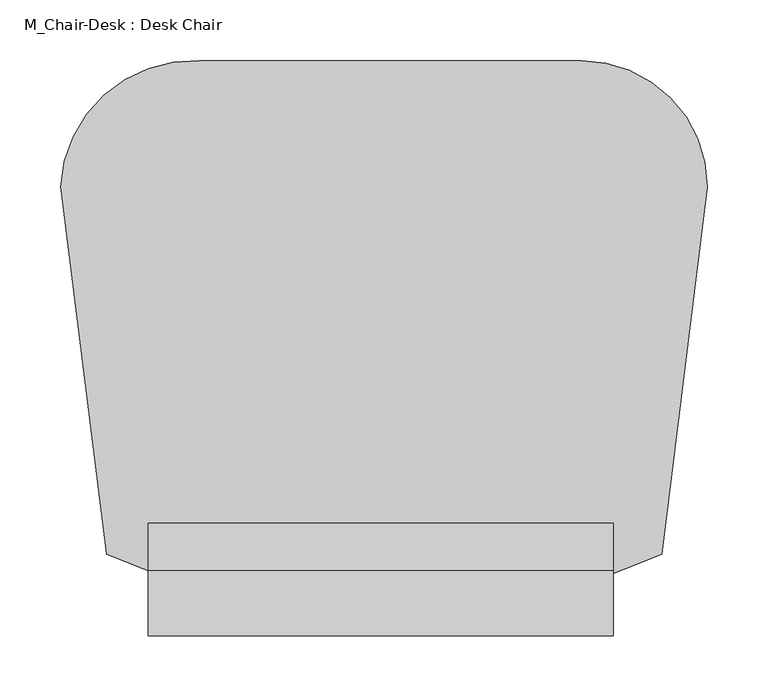
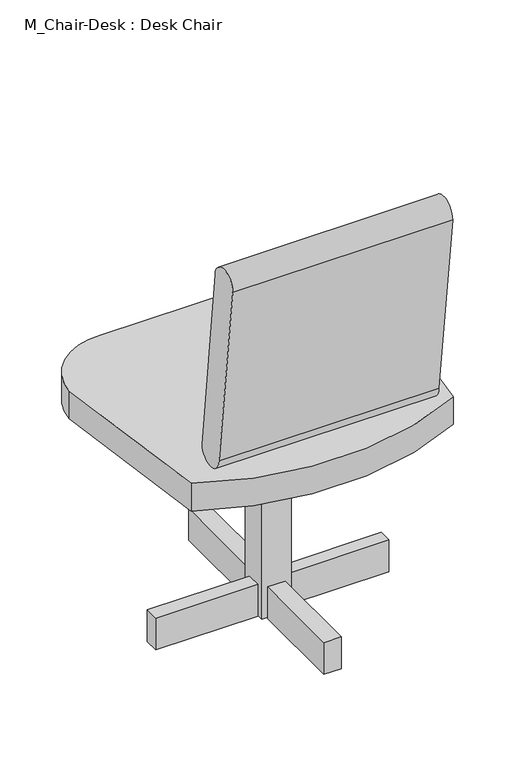
"""IFC4 building model written with IfcOpenShell, lengths in millimetres: furniture geometry, M_Chair-Desk : Desk Chair."""

import ifcopenshell
import ifcopenshell.guid

model = None  # the IFC model being written
_history = None  # IfcOwnerHistory: only IFC2X3 demands one
_inside = {}  # id of a spatial element -> (the spatial element, [elements in it])
_under = {}  # id of a project, library or spatial element -> (it, [spatial elements below it])
_declared = {}  # id of a project -> (the project, [libraries it declares])
_typed = {}  # id of a type object -> (the type object, [elements of that type])
_made_of = {}  # id of a material, layer set ... -> (it, [elements and type objects made of it])


def new_model(schema):
    """Start an empty IFC model of exactly this schema.

    Asked for "IFC4X3", IfcOpenShell would pick the latest addendum, in which some entities
    have other attributes; the version numbers below select the first issue.
    IFC2X3 requires an IfcOwnerHistory on every rooted entity: one is made here for all.
    """
    global model, _history
    if schema == "IFC4X3":
        model = ifcopenshell.file(schema_version=(4, 3, 0, 0))
    else:
        model = ifcopenshell.file(schema=schema)
    _inside.clear()
    _under.clear()
    _declared.clear()
    _typed.clear()
    _made_of.clear()
    _history = None
    if model.schema == "IFC2X3":
        org = make("IfcOrganization", Name="unknown")
        user = make(
            "IfcPersonAndOrganization",
            ThePerson=make("IfcPerson", FamilyName="unknown"),
            TheOrganization=org,
        )
        app = make(
            "IfcApplication",
            ApplicationDeveloper=org,
            Version="unknown",
            ApplicationFullName="unknown",
            ApplicationIdentifier="unknown",
        )
        _history = make(
            "IfcOwnerHistory",
            OwningUser=user,
            OwningApplication=app,
            ChangeAction="ADDED",
            CreationDate=0,
        )
    return model


def make(cls, **values):
    """One entity of the class cls with the attributes given. An attribute that is None is left unset."""
    return model.create_entity(
        cls, **{name: value for name, value in values.items() if value is not None}
    )


def rooted(cls, **values):
    """An entity with a GlobalId (a new one), such as an element, a storey or a relation."""
    return make(cls, GlobalId=ifcopenshell.guid.new(), OwnerHistory=_history, **values)


def si_unit(unit_type, name, prefix=None):
    """IfcSIUnit, for example si_unit("LENGTHUNIT", "METRE", prefix="MILLI")."""
    return make("IfcSIUnit", UnitType=unit_type, Prefix=prefix, Name=name)


def assignment(units):
    """IfcUnitAssignment: the units of a project."""
    return None if units is None else make("IfcUnitAssignment", Units=units)


def point(xyz):
    """IfcCartesianPoint."""
    return None if xyz is None else make("IfcCartesianPoint", Coordinates=xyz)


def direction(xyz):
    """IfcDirection."""
    return None if xyz is None else make("IfcDirection", DirectionRatios=xyz)


def frame(location, z_axis=None, x_axis=None):
    """IfcAxis2Placement3D, a coordinate frame: its origin and axes. An axis left out is left unset."""
    return make(
        "IfcAxis2Placement3D",
        Location=point(location),
        Axis=direction(z_axis),
        RefDirection=direction(x_axis),
    )


def frame_2d(location, x_axis=None):
    """IfcAxis2Placement2D, a coordinate frame in the plane: its origin and x axis."""
    return make(
        "IfcAxis2Placement2D", Location=point(location), RefDirection=direction(x_axis)
    )


def origin():
    """The frame at (0, 0, 0) with its axes left unset."""
    return frame((0.0, 0.0, 0.0))


def origin_with_axes():
    """The frame at (0, 0, 0) with the z axis (0, 0, 1) and the x axis (1, 0, 0) written out."""
    return frame((0.0, 0.0, 0.0), z_axis=(0.0, 0.0, 1.0), x_axis=(1.0, 0.0, 0.0))


def place(relative_to, where):
    """IfcLocalPlacement: puts the frame where relative to a parent placement (None: the world)."""
    return make(
        "IfcLocalPlacement", PlacementRelTo=relative_to, RelativePlacement=where
    )


def context(
    kind, dimensions, precision=None, world=None, true_north=None, identifier=None
):
    """IfcGeometricRepresentationContext, for example the 3D "Model" context."""
    return make(
        "IfcGeometricRepresentationContext",
        ContextIdentifier=identifier,
        ContextType=kind,
        CoordinateSpaceDimension=dimensions,
        Precision=precision,
        WorldCoordinateSystem=world,
        TrueNorth=true_north,
    )


def project(units=None, contexts=None):
    """IfcProject with its units and contexts."""
    return rooted(
        "IfcProject",
        Name="project",
        RepresentationContexts=contexts,
        UnitsInContext=assignment(units),
    )


def spatial(cls, under=None, at=None, **own):
    """A site, building, storey or space (cls), placed at a placement, below another one or the project."""
    s = rooted(cls, ObjectPlacement=at, **own)
    if under is not None:
        _under.setdefault(under.id(), (under, []))[1].append(s)
    return s


def polyline(points):
    """IfcPolyline through the points."""
    return make("IfcPolyline", Points=[point(p) for p in points])


def circle_curve(where, radius):
    """IfcCircle in the frame where."""
    return make("IfcCircle", Position=where, Radius=radius)


def trimmed(basis, trim1, trim2, sense, master):
    """IfcTrimmedCurve: the piece of a basis curve between two trims."""
    return make(
        "IfcTrimmedCurve",
        BasisCurve=basis,
        Trim1=trim1,
        Trim2=trim2,
        SenseAgreement=sense,
        MasterRepresentation=master,
    )


def segment(curve, same_sense, transition):
    """IfcCompositeCurveSegment."""
    return make(
        "IfcCompositeCurveSegment",
        Transition=transition,
        SameSense=same_sense,
        ParentCurve=curve,
    )


def composite_curve(segments, self_intersect=None):
    """IfcCompositeCurve: segments joined end to end."""
    return make("IfcCompositeCurve", Segments=segments, SelfIntersect=self_intersect)


def outline(outer, holes=None, kind="AREA"):
    """IfcArbitraryClosedProfileDef: a profile drawn as a closed curve; with holes, ...WithVoids."""
    if holes is None:
        return make("IfcArbitraryClosedProfileDef", ProfileType=kind, OuterCurve=outer)
    return make(
        "IfcArbitraryProfileDefWithVoids",
        ProfileType=kind,
        OuterCurve=outer,
        InnerCurves=holes,
    )


def extrude(swept, where, along, depth):
    """IfcExtrudedAreaSolid: the profile swept, set in the frame where, extruded along a direction by depth."""
    return make(
        "IfcExtrudedAreaSolid",
        SweptArea=swept,
        Position=where,
        ExtrudedDirection=direction(along),
        Depth=depth,
    )


def shape(context_of_items, identifier, shape_type, items):
    """IfcShapeRepresentation: the items that make up one representation, for example the "Body"."""
    return make(
        "IfcShapeRepresentation",
        ContextOfItems=context_of_items,
        RepresentationIdentifier=identifier,
        RepresentationType=shape_type,
        Items=items,
    )


def source(mapping_origin, context_of_items, identifier, shape_type, items):
    """IfcRepresentationMap: a shape defined once, which mapped items show again and again."""
    return make(
        "IfcRepresentationMap",
        MappingOrigin=mapping_origin,
        MappedRepresentation=shape(context_of_items, identifier, shape_type, items),
    )


def transform(
    local_origin,
    x_axis=None,
    y_axis=None,
    z_axis=None,
    scale=None,
    scale2=None,
    scale3=None,
    uniform=True,
):
    """IfcCartesianTransformationOperator3D, or its non-uniform kind. x_axis, y_axis, z_axis: its Axis1, 2, 3."""
    if uniform:
        return make(
            "IfcCartesianTransformationOperator3D",
            Axis1=direction(x_axis),
            Axis2=direction(y_axis),
            LocalOrigin=point(local_origin),
            Scale=scale,
            Axis3=direction(z_axis),
        )
    return make(
        "IfcCartesianTransformationOperator3DnonUniform",
        Axis1=direction(x_axis),
        Axis2=direction(y_axis),
        LocalOrigin=point(local_origin),
        Scale=scale,
        Axis3=direction(z_axis),
        Scale2=scale2,
        Scale3=scale3,
    )


def mapped(mapping_source, mapping_target):
    """IfcMappedItem: shows the shape of a source again, moved by a transform."""
    return make(
        "IfcMappedItem", MappingSource=mapping_source, MappingTarget=mapping_target
    )


def made_of(thing, what):
    """Note that an element or type object is made of a material, layer set ...; save() writes the relation."""
    if what is not None:
        _made_of.setdefault(what.id(), (what, []))[1].append(thing)
    return thing


def element(
    cls,
    number,
    at=None,
    inside=None,
    cuts=None,
    type_object=None,
    material=None,
    context=None,
    identifier="Body",
    shape_type=None,
    held_by="IfcProductDefinitionShape",
    body=None,
    shapes=None,
    **own,
):
    """One element of the class cls, such as IfcWall. Its Tag is "e" and its number.

    at: its placement. inside: the storey or other place that contains it. cuts: it is an
    opening in that element (IfcRelVoidsElement). A single representation is given by context,
    identifier, shape_type and body (its items); several are given by shapes. held_by: the class
    of the entity that holds the representations. save() writes the other relations.
    """
    e = rooted(cls, Tag="e%d" % number, ObjectPlacement=at, **own)
    if body is not None:
        shapes = [shape(context, identifier, shape_type, body)]
    if shapes is not None:
        e.Representation = make(held_by, Representations=shapes)
    if inside is not None:
        _inside.setdefault(inside.id(), (inside, []))[1].append(e)
    if cuts is not None:
        rooted(
            "IfcRelVoidsElement", RelatingBuildingElement=cuts, RelatedOpeningElement=e
        )
    if type_object is not None:
        _typed.setdefault(type_object.id(), (type_object, []))[1].append(e)
    return made_of(e, material)


def aggregate(whole, parts):
    """IfcRelAggregates: a whole, such as a stair, and the parts it consists of."""
    return rooted("IfcRelAggregates", RelatingObject=whole, RelatedObjects=parts)


def save(model, path):
    """Write the relations noted so far, then the file.

    IfcRelAggregates (storeys below a building ...), IfcRelContainedInSpatialStructure (elements
    in a storey), IfcRelDefinesByType, IfcRelAssociatesMaterial and IfcRelDeclares: one each for
    every whole, place, type object, material and project.
    """
    for whole, parts in _under.values():
        aggregate(whole, parts)
    for where, things in _inside.values():
        rooted(
            "IfcRelContainedInSpatialStructure",
            RelatedElements=things,
            RelatingStructure=where,
        )
    for kind, things in _typed.values():
        rooted("IfcRelDefinesByType", RelatedObjects=things, RelatingType=kind)
    for what, things in _made_of.values():
        rooted("IfcRelAssociatesMaterial", RelatedObjects=things, RelatingMaterial=what)
    for by, libraries in _declared.values():
        rooted("IfcRelDeclares", RelatingContext=by, RelatedDefinitions=libraries)
    model.write(path)


def m_chair_desk_desk_chair_ccc35c8f(model_context):
    return source(origin(), model_context, "Body", "SweptSolid", [
        extrude(outline(polyline([(-203.6618182, 175.0290909), (-25.8618182, 175.0290909), (-25.8618182, 150.0462968), (-203.6618182, 150.0462968), (-203.6618182, 175.0290909)])), origin_with_axes(), (0.0, 0.0, 1.0), 58.5040426),
        extrude(outline(polyline([(204.1236364, 175.0290909), (204.1236364, 152.4), (26.7854545, 152.4), (26.7854545, 175.0290909), (204.1236364, 175.0290909)])), origin_with_axes(), (0.0, 0.0, 1.0), 58.5040426),
        extrude(outline(polyline([(-16.1636364, 188.8836364), (-16.1636364, 374.9517514), (14.3163636, 374.9517514), (14.3163636, 188.8836364), (-16.1636364, 188.8836364)])), origin_with_axes(), (0.0, 0.0, 1.0), 58.5040426),
        extrude(outline(polyline([(14.3163636, 136.2363636), (14.3163636, -33.2509091), (-16.1636364, -33.2509091), (-16.1636364, 136.2363636), (14.3163636, 136.2363636)])), origin_with_axes(), (0.0, 0.0, 1.0), 58.5040426),
        extrude(outline(polyline([(26.3236364, 190.2690909), (26.3236364, 139.4690909), (-24.4763636, 139.4690909), (-24.4763636, 190.2690909), (26.3236364, 190.2690909)])), origin_with_axes(), (0.0, 0.0, 1.0), 355.6),
        extrude(outline(composite_curve([segment(polyline([(-13.6321252, 787.4), (25.5523927, 451.3880753)]), True, "CONTINUOUS"), segment(trimmed(circle_curve(frame_2d((0.0761963, 451.3880753)), 25.4761963), [point((25.5523927, 451.3880753))], [point((-25.4, 451.3880753))], False, "CARTESIAN"), True, "CONTINUOUS"), segment(polyline([(-25.4, 451.3880753), (-67.209111, 787.4)]), True, "CONTINUOUS"), segment(trimmed(circle_curve(frame_2d((-40.4206181, 787.4)), 26.7884929), [point((-67.209111, 787.4))], [point((-13.6321252, 787.4))], False, "CARTESIAN"), True, "CONTINUOUS")], self_intersect=False)), frame((-194.3643056, 0.0, 0.0), z_axis=(1.0, 0.0, 0.0), x_axis=(0.0, 1.0, 0.0)), (0.0, 0.0, 1.0), 383.2768056),
        extrude(outline(composite_curve([segment(trimmed(circle_curve(frame_2d((-157.1362322, 297.1024212)), 109.4001491), [point((-266.4057871, 302.4462968))], [point((-152.4, 406.4))], False, "CARTESIAN"), True, "CONTINUOUS"), segment(polyline([(-152.4, 406.4), (162.2530084, 406.4)]), True, "CONTINUOUS"), segment(trimmed(circle_curve(frame_2d((162.2530084, 302.4462968)), 103.9537032), [point((162.2530084, 406.4))], [point((266.2067116, 302.4462968))], False, "CARTESIAN"), True, "CONTINUOUS"), segment(polyline([(266.2067116, 302.4462968), (228.6, 0.0)]), True, "CONTINUOUS"), segment(trimmed(circle_curve(frame_2d((0.0, 446.8941036)), 501.9684252), [point((228.6, 0.0))], [point((-228.6, 0.0))], False, "CARTESIAN"), True, "CONTINUOUS"), segment(polyline([(-228.6, 0.0), (-266.4057871, 302.4462968)]), True, "CONTINUOUS")], self_intersect=False)), frame((0.0, 0.0, 355.6), z_axis=(0.0, 0.0, 1.0), x_axis=(1.0, 0.0, 0.0)), (0.0, 0.0, 1.0), 50.8),
    ])


if __name__ == "__main__":
    model = new_model("IFC4")
    model_context = context("Model", 3, world=origin())
    ifc_project = project(units=[si_unit("LENGTHUNIT", "METRE", prefix="MILLI")], contexts=[model_context])
    site = spatial("IfcSite", under=ifc_project)
    building = spatial("IfcBuilding", under=site)
    placement = place(None, origin())
    m_chair_desk_desk_chair_shape = m_chair_desk_desk_chair_ccc35c8f(model_context)
    element("IfcFurniture", 1, ObjectType="M_Chair-Desk : Desk Chair", at=placement, inside=building, context=model_context, shape_type="MappedRepresentation", body=[
        mapped(m_chair_desk_desk_chair_shape, transform((0.0, 0.0, 0.0), x_axis=(1.0, 0.0, 0.0), y_axis=(0.0, 1.0, 0.0), z_axis=(0.0, 0.0, 1.0))),
    ])
    save(model, "model.ifc")

# Revit data of these elements
# Type "M_Chair-Desk : Desk Chair"
#   Seat/Back Material = Textile - Slate Blue
#   Base Material = Steel, Chrome Plated
# Element 1 (IfcFurniture, "M_Chair-Desk : Desk Chair")
#   Materials on its faces: "Steel, Chrome Plated", "Textile - Slate Blue"
# Materials
#   "Textile - Slate Blue": class "Fabric", colour RGB 98 102 118, transparency 0
#   "Steel, Chrome Plated": class "Metal", colour RGB 244 244 244, transparency 0, Description = "Chromiuim plated steel", Cost = 0
